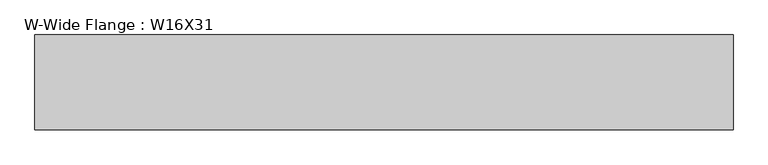
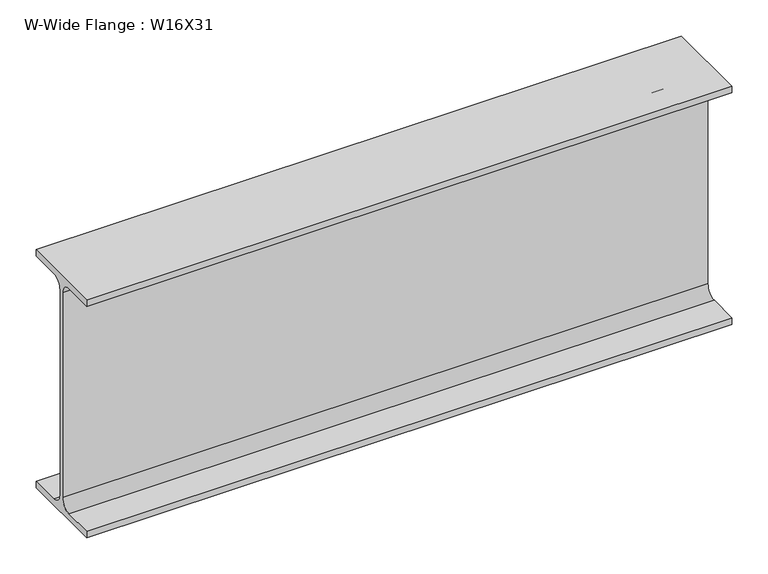
"""IFC4 building model written with IfcOpenShell, lengths in millimetres: beam geometry, W-Wide Flange : W16X31."""

from ifc_helpers import new_model, si_unit, point, frame, frame_2d, origin, place, context, project, spatial, polyline, circle_curve, trimmed, segment, composite_curve, outline, extrude, source, transform, mapped, element, save


def w_wide_flange_w16x31_2e755f9a(model_context):
    return source(origin(), model_context, "Body", "SweptSolid", [
        extrude(outline(composite_curve([segment(polyline([(70.231, -190.754), (70.231, -201.93), (-70.231, -201.93), (-70.231, -190.754), (-20.8915, -190.754)]), True, "CONTINUOUS"), segment(trimmed(circle_curve(frame_2d((-20.8915, -173.355)), 17.399), [point((-20.8915, -190.754))], [point((-3.4925, -173.355))], True, "CARTESIAN"), True, "CONTINUOUS"), segment(polyline([(-3.4925, -173.355), (-3.4925, 173.355)]), True, "CONTINUOUS"), segment(trimmed(circle_curve(frame_2d((-20.8915, 173.355)), 17.399), [point((-3.4925, 173.355))], [point((-20.8915, 190.754))], True, "CARTESIAN"), True, "CONTINUOUS"), segment(polyline([(-20.8915, 190.754), (-70.231, 190.754), (-70.231, 201.93), (70.231, 201.93), (70.231, 190.754), (20.8915, 190.754)]), True, "CONTINUOUS"), segment(trimmed(circle_curve(frame_2d((20.8915, 173.355)), 17.399), [point((20.8915, 190.754))], [point((3.4925, 173.355))], True, "CARTESIAN"), True, "CONTINUOUS"), segment(polyline([(3.4925, 173.355), (3.4925, -173.355)]), True, "CONTINUOUS"), segment(trimmed(circle_curve(frame_2d((20.8915, -173.355)), 17.399), [point((3.4925, -173.355))], [point((20.8915, -190.754))], True, "CARTESIAN"), True, "CONTINUOUS"), segment(polyline([(20.8915, -190.754), (70.231, -190.754)]), True, "CONTINUOUS")], self_intersect=False)), frame((-509.7879677, 0.0, 0.0), z_axis=(1.0, 0.0, 0.0), x_axis=(0.0, 1.0, 0.0)), (0.0, 0.0, 1.0), 1033.9835215),
    ])


if __name__ == "__main__":
    model = new_model("IFC4")
    model_context = context("Model", 3, world=origin())
    ifc_project = project(units=[si_unit("LENGTHUNIT", "METRE", prefix="MILLI")], contexts=[model_context])
    site = spatial("IfcSite", under=ifc_project)
    building = spatial("IfcBuilding", under=site)
    placement = place(None, origin())
    w_wide_flange_w16x31_shape = w_wide_flange_w16x31_2e755f9a(model_context)
    element("IfcBeam", 1, ObjectType="W-Wide Flange : W16X31", at=placement, inside=building, context=model_context, shape_type="MappedRepresentation", body=[
        mapped(w_wide_flange_w16x31_shape, transform((0.0, 0.0, 0.0), x_axis=(1.0, 0.0, 0.0), y_axis=(0.0, 1.0, 0.0), z_axis=(0.0, 0.0, 1.0))),
    ])
    save(model, "model.ifc")

# Revit data of these elements
# Type "W-Wide Flange : W16X31"
#   Assembly Code = "B10"
#   W = 31
#   Start Extension Calculation [instance default] = 10' - 0"
#   Start Extension [instance default] = -0' - 0 1/2"
#   End Extension Calculation [instance default] = 10' - 0"
#   End Extension [instance default] = -0' - 0 1/2"
#   Length [instance default] = 5' - 0"
#   bf = 0' - 5.53"
#   d = 1' - 3.9"
#   k = 0' - 1 1/8"
#   k2 = 0' - 0.685"
#   tf = 0' - 0.44"
#   tw = 0' - 0.275"
#   A = 0.0634028 SF
#   Beam Material [instance default] = Metal - Steel - ASTM A992
# Element 1 (IfcBeam, "W-Wide Flange : W16X31")
#   Materials on its faces: "Metal - Steel - ASTM A992"
# Materials
#   "Metal - Steel - ASTM A992": class "Metal", colour RGB 128 0 0, transparency 0
